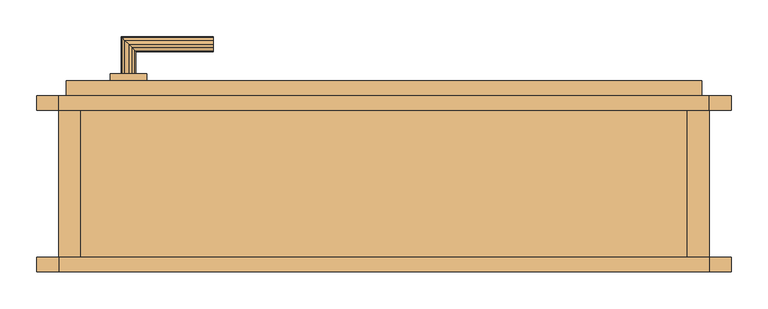
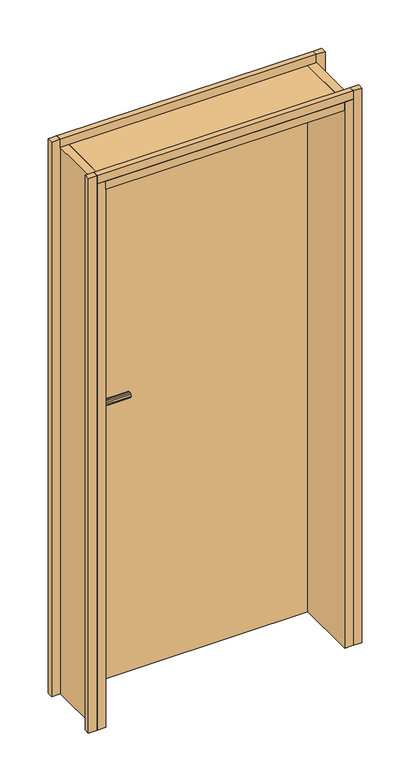
"""IFC4 building model written with IfcOpenShell, lengths in millimetres: door geometry, Tür."""

from ifc_helpers import new_model, si_unit, frame, origin, place, context, project, spatial, polyline, outline, extrude, faceted_brep, source, transform, mapped, element, save


def door_46cdb682(model_context):
    return source(origin(), model_context, "Body", "SolidModel", [
        faceted_brep([(90.0, 190.0, 1198.660254), (95.0, 190.0, 1200.0), (100.0, 190.0, 1198.660254), (103.660254, 190.0, 1195.0), (105.0, 190.0, 1190.0), (103.660254, 190.0, 1185.0), (100.0, 190.0, 1181.339746), (95.0, 190.0, 1180.0), (90.0, 190.0, 1181.339746), (86.339746, 190.0, 1185.0), (85.0, 190.0, 1190.0), (86.339746, 190.0, 1195.0), (95.0, 150.0, 1200.0), (90.0, 145.0, 1198.660254), (86.339746, 141.339746, 1195.0), (85.0, 140.0, 1190.0), (86.339746, 141.339746, 1185.0), (90.0, 145.0, 1181.339746), (95.0, 150.0, 1180.0), (100.0, 155.0, 1181.339746), (103.660254, 158.660254, 1185.0), (105.0, 160.0, 1190.0), (103.660254, 158.660254, 1195.0), (100.0, 155.0, 1198.660254), (210.0, 155.0, 1198.660254), (210.0, 150.0, 1200.0), (210.0, 145.0, 1198.660254), (210.0, 141.339746, 1195.0), (210.0, 140.0, 1190.0), (210.0, 141.339746, 1185.0), (210.0, 145.0, 1181.339746), (210.0, 150.0, 1180.0), (210.0, 155.0, 1181.339746), (210.0, 158.660254, 1185.0), (210.0, 160.0, 1190.0), (210.0, 158.660254, 1195.0)], [[[0, 1, 2, 3, 4, 5, 6, 7, 8, 9, 10, 11]], [[12, 1, 0, 13]], [[13, 0, 11, 14]], [[14, 11, 10, 15]], [[15, 10, 9, 16]], [[16, 9, 8, 17]], [[17, 8, 7, 18]], [[18, 7, 6, 19]], [[19, 6, 5, 20]], [[20, 5, 4, 21]], [[21, 4, 3, 22]], [[22, 3, 2, 23]], [[23, 2, 1, 12]], [[24, 25, 26, 27, 28, 29, 30, 31, 32, 33, 34, 35]], [[25, 12, 13, 26]], [[26, 13, 14, 27]], [[27, 14, 15, 28]], [[28, 15, 16, 29]], [[29, 16, 17, 30]], [[30, 17, 18, 31]], [[31, 18, 19, 32]], [[32, 19, 20, 33]], [[33, 20, 21, 34]], [[34, 21, 22, 35]], [[35, 22, 23, 24]], [[24, 23, 12, 25]]]),
        extrude(outline(polyline([(0.0, -20.0), (-30.0, -20.0), (-30.0, 0.0), (0.0, 0.0), (0.0, -20.0)])), frame((0.0, 0.0, 140.0), z_axis=(0.0, 0.0, 1.0), x_axis=(1.0, 0.0, 0.0)), (0.0, 0.0, 1.0), 2025.0),
        extrude(outline(polyline([(885.0, -20.0), (855.0, -20.0), (855.0, 220.0), (885.0, 220.0), (885.0, -20.0)])), frame((0.0, 0.0, 140.0), z_axis=(0.0, 0.0, 1.0), x_axis=(1.0, 0.0, 0.0)), (0.0, 0.0, 1.0), 1995.0),
        extrude(outline(polyline([(915.0, 220.0), (915.0, 200.0), (885.0, 200.0), (885.0, 220.0), (915.0, 220.0)])), frame((0.0, 0.0, 140.0), z_axis=(0.0, 0.0, 1.0), x_axis=(1.0, 0.0, 0.0)), (0.0, 0.0, 1.0), 2025.0),
        extrude(outline(polyline([(885.0, 200.0), (0.0, 200.0), (0.0, 220.0), (885.0, 220.0), (885.0, 200.0)])), frame((0.0, 0.0, 2135.0), z_axis=(0.0, 0.0, 1.0), x_axis=(1.0, 0.0, 0.0)), (0.0, 0.0, 1.0), 30.0),
        extrude(outline(polyline([(885.0, -20.0), (0.0, -20.0), (0.0, 0.0), (885.0, 0.0), (885.0, -20.0)])), frame((0.0, 0.0, 2135.0), z_axis=(0.0, 0.0, 1.0), x_axis=(1.0, 0.0, 0.0)), (0.0, 0.0, 1.0), 30.0),
        faceted_brep([(100.0, 250.0, 1198.660254), (95.0, 250.0, 1200.0), (90.0, 250.0, 1198.660254), (86.339746, 250.0, 1195.0), (85.0, 250.0, 1190.0), (86.339746, 250.0, 1185.0), (90.0, 250.0, 1181.339746), (95.0, 250.0, 1180.0), (100.0, 250.0, 1181.339746), (103.660254, 250.0, 1185.0), (105.0, 250.0, 1190.0), (103.660254, 250.0, 1195.0), (95.0, 290.0, 1200.0), (90.0, 295.0, 1198.660254), (86.339746, 298.660254, 1195.0), (85.0, 300.0, 1190.0), (86.339746, 298.660254, 1185.0), (90.0, 295.0, 1181.339746), (95.0, 290.0, 1180.0), (100.0, 285.0, 1181.339746), (103.660254, 281.339746, 1185.0), (105.0, 280.0, 1190.0), (103.660254, 281.339746, 1195.0), (100.0, 285.0, 1198.660254), (210.0, 295.0, 1198.660254), (210.0, 290.0, 1200.0), (210.0, 285.0, 1198.660254), (210.0, 281.339746, 1195.0), (210.0, 280.0, 1190.0), (210.0, 281.339746, 1185.0), (210.0, 285.0, 1181.339746), (210.0, 290.0, 1180.0), (210.0, 295.0, 1181.339746), (210.0, 298.660254, 1185.0), (210.0, 300.0, 1190.0), (210.0, 298.660254, 1195.0)], [[[0, 1, 2, 3, 4, 5, 6, 7, 8, 9, 10, 11]], [[2, 1, 12, 13]], [[3, 2, 13, 14]], [[4, 3, 14, 15]], [[5, 4, 15, 16]], [[6, 5, 16, 17]], [[7, 6, 17, 18]], [[8, 7, 18, 19]], [[9, 8, 19, 20]], [[10, 9, 20, 21]], [[11, 10, 21, 22]], [[0, 11, 22, 23]], [[1, 0, 23, 12]], [[24, 25, 26, 27, 28, 29, 30, 31, 32, 33, 34, 35]], [[13, 12, 25, 24]], [[14, 13, 24, 35]], [[15, 14, 35, 34]], [[16, 15, 34, 33]], [[17, 16, 33, 32]], [[18, 17, 32, 31]], [[19, 18, 31, 30]], [[20, 19, 30, 29]], [[21, 20, 29, 28]], [[22, 21, 28, 27]], [[23, 22, 27, 26]], [[12, 23, 26, 25]]]),
        extrude(outline(polyline([(875.0, 200.0), (10.0, 200.0), (10.0, 240.0), (875.0, 240.0), (875.0, 200.0)])), frame((0.0, 0.0, 140.0), z_axis=(0.0, 0.0, 1.0), x_axis=(1.0, 0.0, 0.0)), (0.0, 0.0, 1.0), 1985.0),
        extrude(outline(polyline([(855.0, -20.0), (30.0, -20.0), (30.0, 220.0), (855.0, 220.0), (855.0, -20.0)])), frame((0.0, 0.0, 2105.0), z_axis=(0.0, 0.0, 1.0), x_axis=(1.0, 0.0, 0.0)), (0.0, 0.0, 1.0), 30.0),
        extrude(outline(polyline([(120.0, 240.0), (70.0, 240.0), (70.0, 250.0), (120.0, 250.0), (120.0, 240.0)])), frame((0.0, 0.0, 1050.0), z_axis=(0.0, 0.0, 1.0), x_axis=(1.0, 0.0, 0.0)), (0.0, 0.0, 1.0), 215.0),
        extrude(outline(polyline([(0.0, 200.0), (-30.0, 200.0), (-30.0, 220.0), (0.0, 220.0), (0.0, 200.0)])), frame((0.0, 0.0, 140.0), z_axis=(0.0, 0.0, 1.0), x_axis=(1.0, 0.0, 0.0)), (0.0, 0.0, 1.0), 2025.0),
        extrude(outline(polyline([(915.0, 0.0), (915.0, -20.0), (885.0, -20.0), (885.0, 0.0), (915.0, 0.0)])), frame((0.0, 0.0, 140.0), z_axis=(0.0, 0.0, 1.0), x_axis=(1.0, 0.0, 0.0)), (0.0, 0.0, 1.0), 2025.0),
        extrude(outline(polyline([(30.0, -20.0), (0.0, -20.0), (0.0, 220.0), (30.0, 220.0), (30.0, -20.0)])), frame((0.0, 0.0, 140.0), z_axis=(0.0, 0.0, 1.0), x_axis=(1.0, 0.0, 0.0)), (0.0, 0.0, 1.0), 1995.0),
        extrude(outline(polyline([(70.0, 190.0), (70.0, 200.0), (120.0, 200.0), (120.0, 190.0), (70.0, 190.0)])), frame((0.0, 0.0, 1050.0), z_axis=(0.0, 0.0, 1.0), x_axis=(1.0, 0.0, 0.0)), (0.0, 0.0, 1.0), 215.0),
    ])


if __name__ == "__main__":
    model = new_model("IFC4")
    model_context = context("Model", 3, world=origin())
    ifc_project = project(units=[si_unit("LENGTHUNIT", "METRE", prefix="MILLI")], contexts=[model_context])
    site = spatial("IfcSite", under=ifc_project)
    building = spatial("IfcBuilding", under=site)
    placement = place(None, origin())
    door_shape = door_46cdb682(model_context)
    element("IfcDoor", 1, ObjectType="Tür", at=placement, inside=building, context=model_context, shape_type="MappedRepresentation", body=[
        mapped(door_shape, transform((0.0, 0.0, 0.0), x_axis=(1.0, 0.0, 0.0), y_axis=(0.0, 1.0, 0.0), z_axis=(0.0, 0.0, 1.0))),
    ])
    save(model, "model.ifc")

# Revit data of these elements
# Type "Tür"
#   Type Mark = "32"
# Element 1 (IfcDoor, "Tür")
#   Materials on its faces: "tuer_beschlag", "tuer_holzzarge"
# Materials
#   "tuer_beschlag": class "Unassigned", colour RGB 128 128 128, transparency 0
#   "tuer_holzzarge": class "Unassigned", colour RGB 255 255 255, transparency 0
